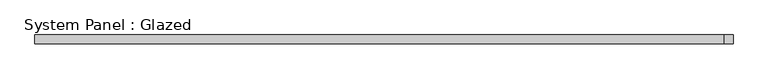
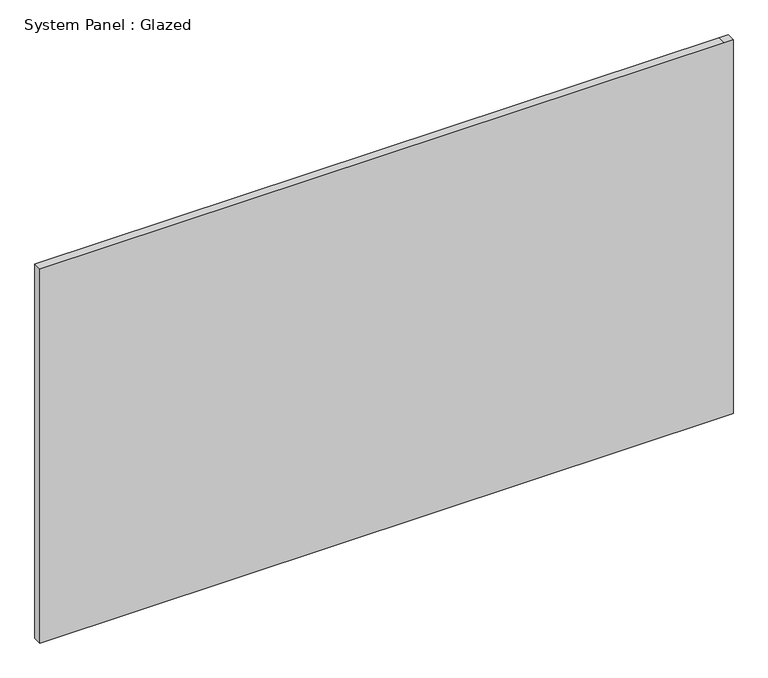
"""IFC4 building model written with IfcOpenShell, lengths in millimetres: plate geometry, System Panel : Glazed."""

import ifcopenshell
import ifcopenshell.guid

model = None  # the IFC model being written
_history = None  # IfcOwnerHistory: only IFC2X3 demands one
_inside = {}  # id of a spatial element -> (the spatial element, [elements in it])
_under = {}  # id of a project, library or spatial element -> (it, [spatial elements below it])
_declared = {}  # id of a project -> (the project, [libraries it declares])
_typed = {}  # id of a type object -> (the type object, [elements of that type])
_made_of = {}  # id of a material, layer set ... -> (it, [elements and type objects made of it])


def new_model(schema):
    """Start an empty IFC model of exactly this schema.

    Asked for "IFC4X3", IfcOpenShell would pick the latest addendum, in which some entities
    have other attributes; the version numbers below select the first issue.
    IFC2X3 requires an IfcOwnerHistory on every rooted entity: one is made here for all.
    """
    global model, _history
    if schema == "IFC4X3":
        model = ifcopenshell.file(schema_version=(4, 3, 0, 0))
    else:
        model = ifcopenshell.file(schema=schema)
    _inside.clear()
    _under.clear()
    _declared.clear()
    _typed.clear()
    _made_of.clear()
    _history = None
    if model.schema == "IFC2X3":
        org = make("IfcOrganization", Name="unknown")
        user = make(
            "IfcPersonAndOrganization",
            ThePerson=make("IfcPerson", FamilyName="unknown"),
            TheOrganization=org,
        )
        app = make(
            "IfcApplication",
            ApplicationDeveloper=org,
            Version="unknown",
            ApplicationFullName="unknown",
            ApplicationIdentifier="unknown",
        )
        _history = make(
            "IfcOwnerHistory",
            OwningUser=user,
            OwningApplication=app,
            ChangeAction="ADDED",
            CreationDate=0,
        )
    return model


def make(cls, **values):
    """One entity of the class cls with the attributes given. An attribute that is None is left unset."""
    return model.create_entity(
        cls, **{name: value for name, value in values.items() if value is not None}
    )


def rooted(cls, **values):
    """An entity with a GlobalId (a new one), such as an element, a storey or a relation."""
    return make(cls, GlobalId=ifcopenshell.guid.new(), OwnerHistory=_history, **values)


def si_unit(unit_type, name, prefix=None):
    """IfcSIUnit, for example si_unit("LENGTHUNIT", "METRE", prefix="MILLI")."""
    return make("IfcSIUnit", UnitType=unit_type, Prefix=prefix, Name=name)


def assignment(units):
    """IfcUnitAssignment: the units of a project."""
    return None if units is None else make("IfcUnitAssignment", Units=units)


def point(xyz):
    """IfcCartesianPoint."""
    return None if xyz is None else make("IfcCartesianPoint", Coordinates=xyz)


def direction(xyz):
    """IfcDirection."""
    return None if xyz is None else make("IfcDirection", DirectionRatios=xyz)


def frame(location, z_axis=None, x_axis=None):
    """IfcAxis2Placement3D, a coordinate frame: its origin and axes. An axis left out is left unset."""
    return make(
        "IfcAxis2Placement3D",
        Location=point(location),
        Axis=direction(z_axis),
        RefDirection=direction(x_axis),
    )


def origin():
    """The frame at (0, 0, 0) with its axes left unset."""
    return frame((0.0, 0.0, 0.0))


def place(relative_to, where):
    """IfcLocalPlacement: puts the frame where relative to a parent placement (None: the world)."""
    return make(
        "IfcLocalPlacement", PlacementRelTo=relative_to, RelativePlacement=where
    )


def context(
    kind, dimensions, precision=None, world=None, true_north=None, identifier=None
):
    """IfcGeometricRepresentationContext, for example the 3D "Model" context."""
    return make(
        "IfcGeometricRepresentationContext",
        ContextIdentifier=identifier,
        ContextType=kind,
        CoordinateSpaceDimension=dimensions,
        Precision=precision,
        WorldCoordinateSystem=world,
        TrueNorth=true_north,
    )


def project(units=None, contexts=None):
    """IfcProject with its units and contexts."""
    return rooted(
        "IfcProject",
        Name="project",
        RepresentationContexts=contexts,
        UnitsInContext=assignment(units),
    )


def spatial(cls, under=None, at=None, **own):
    """A site, building, storey or space (cls), placed at a placement, below another one or the project."""
    s = rooted(cls, ObjectPlacement=at, **own)
    if under is not None:
        _under.setdefault(under.id(), (under, []))[1].append(s)
    return s


def polyline(points):
    """IfcPolyline through the points."""
    return make("IfcPolyline", Points=[point(p) for p in points])


def outline(outer, holes=None, kind="AREA"):
    """IfcArbitraryClosedProfileDef: a profile drawn as a closed curve; with holes, ...WithVoids."""
    if holes is None:
        return make("IfcArbitraryClosedProfileDef", ProfileType=kind, OuterCurve=outer)
    return make(
        "IfcArbitraryProfileDefWithVoids",
        ProfileType=kind,
        OuterCurve=outer,
        InnerCurves=holes,
    )


def extrude(swept, where, along, depth):
    """IfcExtrudedAreaSolid: the profile swept, set in the frame where, extruded along a direction by depth."""
    return make(
        "IfcExtrudedAreaSolid",
        SweptArea=swept,
        Position=where,
        ExtrudedDirection=direction(along),
        Depth=depth,
    )


def shape(context_of_items, identifier, shape_type, items):
    """IfcShapeRepresentation: the items that make up one representation, for example the "Body"."""
    return make(
        "IfcShapeRepresentation",
        ContextOfItems=context_of_items,
        RepresentationIdentifier=identifier,
        RepresentationType=shape_type,
        Items=items,
    )


def source(mapping_origin, context_of_items, identifier, shape_type, items):
    """IfcRepresentationMap: a shape defined once, which mapped items show again and again."""
    return make(
        "IfcRepresentationMap",
        MappingOrigin=mapping_origin,
        MappedRepresentation=shape(context_of_items, identifier, shape_type, items),
    )


def transform(
    local_origin,
    x_axis=None,
    y_axis=None,
    z_axis=None,
    scale=None,
    scale2=None,
    scale3=None,
    uniform=True,
):
    """IfcCartesianTransformationOperator3D, or its non-uniform kind. x_axis, y_axis, z_axis: its Axis1, 2, 3."""
    if uniform:
        return make(
            "IfcCartesianTransformationOperator3D",
            Axis1=direction(x_axis),
            Axis2=direction(y_axis),
            LocalOrigin=point(local_origin),
            Scale=scale,
            Axis3=direction(z_axis),
        )
    return make(
        "IfcCartesianTransformationOperator3DnonUniform",
        Axis1=direction(x_axis),
        Axis2=direction(y_axis),
        LocalOrigin=point(local_origin),
        Scale=scale,
        Axis3=direction(z_axis),
        Scale2=scale2,
        Scale3=scale3,
    )


def mapped(mapping_source, mapping_target):
    """IfcMappedItem: shows the shape of a source again, moved by a transform."""
    return make(
        "IfcMappedItem", MappingSource=mapping_source, MappingTarget=mapping_target
    )


def made_of(thing, what):
    """Note that an element or type object is made of a material, layer set ...; save() writes the relation."""
    if what is not None:
        _made_of.setdefault(what.id(), (what, []))[1].append(thing)
    return thing


def element(
    cls,
    number,
    at=None,
    inside=None,
    cuts=None,
    type_object=None,
    material=None,
    context=None,
    identifier="Body",
    shape_type=None,
    held_by="IfcProductDefinitionShape",
    body=None,
    shapes=None,
    **own,
):
    """One element of the class cls, such as IfcWall. Its Tag is "e" and its number.

    at: its placement. inside: the storey or other place that contains it. cuts: it is an
    opening in that element (IfcRelVoidsElement). A single representation is given by context,
    identifier, shape_type and body (its items); several are given by shapes. held_by: the class
    of the entity that holds the representations. save() writes the other relations.
    """
    e = rooted(cls, Tag="e%d" % number, ObjectPlacement=at, **own)
    if body is not None:
        shapes = [shape(context, identifier, shape_type, body)]
    if shapes is not None:
        e.Representation = make(held_by, Representations=shapes)
    if inside is not None:
        _inside.setdefault(inside.id(), (inside, []))[1].append(e)
    if cuts is not None:
        rooted(
            "IfcRelVoidsElement", RelatingBuildingElement=cuts, RelatedOpeningElement=e
        )
    if type_object is not None:
        _typed.setdefault(type_object.id(), (type_object, []))[1].append(e)
    return made_of(e, material)


def aggregate(whole, parts):
    """IfcRelAggregates: a whole, such as a stair, and the parts it consists of."""
    return rooted("IfcRelAggregates", RelatingObject=whole, RelatedObjects=parts)


def save(model, path):
    """Write the relations noted so far, then the file.

    IfcRelAggregates (storeys below a building ...), IfcRelContainedInSpatialStructure (elements
    in a storey), IfcRelDefinesByType, IfcRelAssociatesMaterial and IfcRelDeclares: one each for
    every whole, place, type object, material and project.
    """
    for whole, parts in _under.values():
        aggregate(whole, parts)
    for where, things in _inside.values():
        rooted(
            "IfcRelContainedInSpatialStructure",
            RelatedElements=things,
            RelatingStructure=where,
        )
    for kind, things in _typed.values():
        rooted("IfcRelDefinesByType", RelatedObjects=things, RelatingType=kind)
    for what, things in _made_of.values():
        rooted("IfcRelAssociatesMaterial", RelatedObjects=things, RelatingMaterial=what)
    for by, libraries in _declared.values():
        rooted("IfcRelDeclares", RelatingContext=by, RelatedDefinitions=libraries)
    model.write(path)


def system_panel_glazed_75599714(model_context):
    return source(origin(), model_context, "Body", "SweptSolid", [
        extrude(outline(polyline([(0.0, -1012.825), (0.0, 987.425), (0.0, 1012.825), (1155.7, 1012.825), (1155.7, 987.425), (1155.7, -1012.825), (0.0, -1012.825)])), frame((0.0, -44.45, 0.0), z_axis=(0.0, 1.0, 0.0), x_axis=(0.0, 0.0, 1.0)), (0.0, 0.0, 1.0), 25.4),
    ])


if __name__ == "__main__":
    model = new_model("IFC4")
    model_context = context("Model", 3, world=origin())
    ifc_project = project(units=[si_unit("LENGTHUNIT", "METRE", prefix="MILLI")], contexts=[model_context])
    site = spatial("IfcSite", under=ifc_project)
    building = spatial("IfcBuilding", under=site)
    placement = place(None, origin())
    system_panel_glazed_shape = system_panel_glazed_75599714(model_context)
    element("IfcPlate", 1, ObjectType="System Panel : Glazed", at=placement, inside=building, context=model_context, shape_type="MappedRepresentation", body=[
        mapped(system_panel_glazed_shape, transform((0.0, 0.0, 0.0), x_axis=(1.0, 0.0, 0.0), y_axis=(0.0, 1.0, 0.0), z_axis=(0.0, 0.0, 1.0))),
    ])
    save(model, "model.ifc")

# Revit data of these elements
# Element 1 (IfcPlate, "System Panel : Glazed")
#   Materials on its faces: "Glass"
# Materials
#   "Glass": class "Glass", colour RGB 0 128 192, transparency 0.75, Cost = 0
